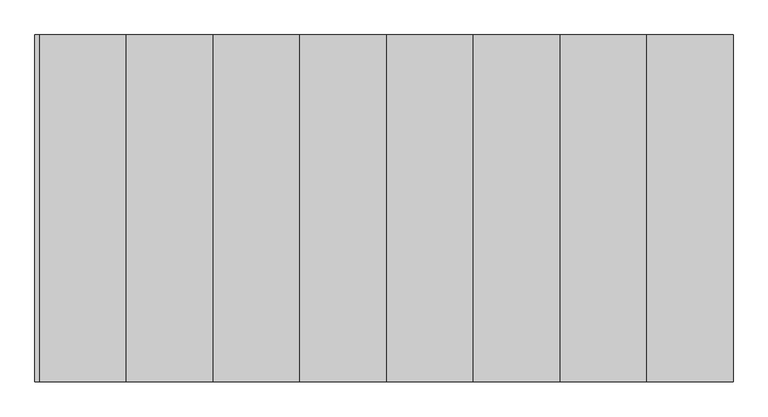
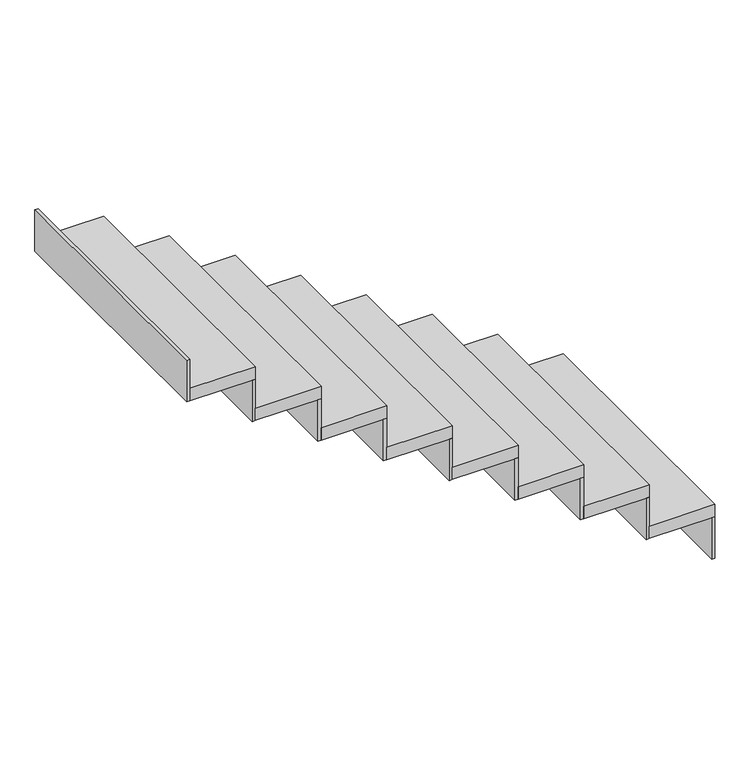
"""IFC4 building model written with IfcOpenShell, lengths in millimetres: stair flight geometry."""

import ifcopenshell
import ifcopenshell.guid

model = None  # the IFC model being written
_history = None  # IfcOwnerHistory: only IFC2X3 demands one
_inside = {}  # id of a spatial element -> (the spatial element, [elements in it])
_under = {}  # id of a project, library or spatial element -> (it, [spatial elements below it])
_declared = {}  # id of a project -> (the project, [libraries it declares])
_typed = {}  # id of a type object -> (the type object, [elements of that type])
_made_of = {}  # id of a material, layer set ... -> (it, [elements and type objects made of it])


def new_model(schema):
    """Start an empty IFC model of exactly this schema.

    Asked for "IFC4X3", IfcOpenShell would pick the latest addendum, in which some entities
    have other attributes; the version numbers below select the first issue.
    IFC2X3 requires an IfcOwnerHistory on every rooted entity: one is made here for all.
    """
    global model, _history
    if schema == "IFC4X3":
        model = ifcopenshell.file(schema_version=(4, 3, 0, 0))
    else:
        model = ifcopenshell.file(schema=schema)
    _inside.clear()
    _under.clear()
    _declared.clear()
    _typed.clear()
    _made_of.clear()
    _history = None
    if model.schema == "IFC2X3":
        org = make("IfcOrganization", Name="unknown")
        user = make(
            "IfcPersonAndOrganization",
            ThePerson=make("IfcPerson", FamilyName="unknown"),
            TheOrganization=org,
        )
        app = make(
            "IfcApplication",
            ApplicationDeveloper=org,
            Version="unknown",
            ApplicationFullName="unknown",
            ApplicationIdentifier="unknown",
        )
        _history = make(
            "IfcOwnerHistory",
            OwningUser=user,
            OwningApplication=app,
            ChangeAction="ADDED",
            CreationDate=0,
        )
    return model


def make(cls, **values):
    """One entity of the class cls with the attributes given. An attribute that is None is left unset."""
    return model.create_entity(
        cls, **{name: value for name, value in values.items() if value is not None}
    )


def rooted(cls, **values):
    """An entity with a GlobalId (a new one), such as an element, a storey or a relation."""
    return make(cls, GlobalId=ifcopenshell.guid.new(), OwnerHistory=_history, **values)


def si_unit(unit_type, name, prefix=None):
    """IfcSIUnit, for example si_unit("LENGTHUNIT", "METRE", prefix="MILLI")."""
    return make("IfcSIUnit", UnitType=unit_type, Prefix=prefix, Name=name)


def assignment(units):
    """IfcUnitAssignment: the units of a project."""
    return None if units is None else make("IfcUnitAssignment", Units=units)


def point(xyz):
    """IfcCartesianPoint."""
    return None if xyz is None else make("IfcCartesianPoint", Coordinates=xyz)


def direction(xyz):
    """IfcDirection."""
    return None if xyz is None else make("IfcDirection", DirectionRatios=xyz)


def frame(location, z_axis=None, x_axis=None):
    """IfcAxis2Placement3D, a coordinate frame: its origin and axes. An axis left out is left unset."""
    return make(
        "IfcAxis2Placement3D",
        Location=point(location),
        Axis=direction(z_axis),
        RefDirection=direction(x_axis),
    )


def origin():
    """The frame at (0, 0, 0) with its axes left unset."""
    return frame((0.0, 0.0, 0.0))


def place(relative_to, where):
    """IfcLocalPlacement: puts the frame where relative to a parent placement (None: the world)."""
    return make(
        "IfcLocalPlacement", PlacementRelTo=relative_to, RelativePlacement=where
    )


def context(
    kind, dimensions, precision=None, world=None, true_north=None, identifier=None
):
    """IfcGeometricRepresentationContext, for example the 3D "Model" context."""
    return make(
        "IfcGeometricRepresentationContext",
        ContextIdentifier=identifier,
        ContextType=kind,
        CoordinateSpaceDimension=dimensions,
        Precision=precision,
        WorldCoordinateSystem=world,
        TrueNorth=true_north,
    )


def project(units=None, contexts=None):
    """IfcProject with its units and contexts."""
    return rooted(
        "IfcProject",
        Name="project",
        RepresentationContexts=contexts,
        UnitsInContext=assignment(units),
    )


def spatial(cls, under=None, at=None, **own):
    """A site, building, storey or space (cls), placed at a placement, below another one or the project."""
    s = rooted(cls, ObjectPlacement=at, **own)
    if under is not None:
        _under.setdefault(under.id(), (under, []))[1].append(s)
    return s


def polyline(points):
    """IfcPolyline through the points."""
    return make("IfcPolyline", Points=[point(p) for p in points])


def outline(outer, holes=None, kind="AREA"):
    """IfcArbitraryClosedProfileDef: a profile drawn as a closed curve; with holes, ...WithVoids."""
    if holes is None:
        return make("IfcArbitraryClosedProfileDef", ProfileType=kind, OuterCurve=outer)
    return make(
        "IfcArbitraryProfileDefWithVoids",
        ProfileType=kind,
        OuterCurve=outer,
        InnerCurves=holes,
    )


def extrude(swept, where, along, depth):
    """IfcExtrudedAreaSolid: the profile swept, set in the frame where, extruded along a direction by depth."""
    return make(
        "IfcExtrudedAreaSolid",
        SweptArea=swept,
        Position=where,
        ExtrudedDirection=direction(along),
        Depth=depth,
    )


def shape(context_of_items, identifier, shape_type, items):
    """IfcShapeRepresentation: the items that make up one representation, for example the "Body"."""
    return make(
        "IfcShapeRepresentation",
        ContextOfItems=context_of_items,
        RepresentationIdentifier=identifier,
        RepresentationType=shape_type,
        Items=items,
    )


def source(mapping_origin, context_of_items, identifier, shape_type, items):
    """IfcRepresentationMap: a shape defined once, which mapped items show again and again."""
    return make(
        "IfcRepresentationMap",
        MappingOrigin=mapping_origin,
        MappedRepresentation=shape(context_of_items, identifier, shape_type, items),
    )


def transform(
    local_origin,
    x_axis=None,
    y_axis=None,
    z_axis=None,
    scale=None,
    scale2=None,
    scale3=None,
    uniform=True,
):
    """IfcCartesianTransformationOperator3D, or its non-uniform kind. x_axis, y_axis, z_axis: its Axis1, 2, 3."""
    if uniform:
        return make(
            "IfcCartesianTransformationOperator3D",
            Axis1=direction(x_axis),
            Axis2=direction(y_axis),
            LocalOrigin=point(local_origin),
            Scale=scale,
            Axis3=direction(z_axis),
        )
    return make(
        "IfcCartesianTransformationOperator3DnonUniform",
        Axis1=direction(x_axis),
        Axis2=direction(y_axis),
        LocalOrigin=point(local_origin),
        Scale=scale,
        Axis3=direction(z_axis),
        Scale2=scale2,
        Scale3=scale3,
    )


def mapped(mapping_source, mapping_target):
    """IfcMappedItem: shows the shape of a source again, moved by a transform."""
    return make(
        "IfcMappedItem", MappingSource=mapping_source, MappingTarget=mapping_target
    )


def made_of(thing, what):
    """Note that an element or type object is made of a material, layer set ...; save() writes the relation."""
    if what is not None:
        _made_of.setdefault(what.id(), (what, []))[1].append(thing)
    return thing


def element(
    cls,
    number,
    at=None,
    inside=None,
    cuts=None,
    type_object=None,
    material=None,
    context=None,
    identifier="Body",
    shape_type=None,
    held_by="IfcProductDefinitionShape",
    body=None,
    shapes=None,
    **own,
):
    """One element of the class cls, such as IfcWall. Its Tag is "e" and its number.

    at: its placement. inside: the storey or other place that contains it. cuts: it is an
    opening in that element (IfcRelVoidsElement). A single representation is given by context,
    identifier, shape_type and body (its items); several are given by shapes. held_by: the class
    of the entity that holds the representations. save() writes the other relations.
    """
    e = rooted(cls, Tag="e%d" % number, ObjectPlacement=at, **own)
    if body is not None:
        shapes = [shape(context, identifier, shape_type, body)]
    if shapes is not None:
        e.Representation = make(held_by, Representations=shapes)
    if inside is not None:
        _inside.setdefault(inside.id(), (inside, []))[1].append(e)
    if cuts is not None:
        rooted(
            "IfcRelVoidsElement", RelatingBuildingElement=cuts, RelatedOpeningElement=e
        )
    if type_object is not None:
        _typed.setdefault(type_object.id(), (type_object, []))[1].append(e)
    return made_of(e, material)


def aggregate(whole, parts):
    """IfcRelAggregates: a whole, such as a stair, and the parts it consists of."""
    return rooted("IfcRelAggregates", RelatingObject=whole, RelatedObjects=parts)


def save(model, path):
    """Write the relations noted so far, then the file.

    IfcRelAggregates (storeys below a building ...), IfcRelContainedInSpatialStructure (elements
    in a storey), IfcRelDefinesByType, IfcRelAssociatesMaterial and IfcRelDeclares: one each for
    every whole, place, type object, material and project.
    """
    for whole, parts in _under.values():
        aggregate(whole, parts)
    for where, things in _inside.values():
        rooted(
            "IfcRelContainedInSpatialStructure",
            RelatedElements=things,
            RelatingStructure=where,
        )
    for kind, things in _typed.values():
        rooted("IfcRelDefinesByType", RelatedObjects=things, RelatingType=kind)
    for what, things in _made_of.values():
        rooted("IfcRelAssociatesMaterial", RelatedObjects=things, RelatingMaterial=what)
    for by, libraries in _declared.values():
        rooted("IfcRelDeclares", RelatingContext=by, RelatedDefinitions=libraries)
    model.write(path)


def stair_flight_f3270307(model_context):
    return source(origin(), model_context, "Body", "SweptSolid", [
        extrude(outline(polyline([(5264.0556606, 2510.81281), (5276.5556606, 2510.81281), (5276.5556606, 1510.81281), (5264.0556606, 1510.81281), (5264.0556606, 2510.81281)])), frame((0.0, 0.0, 4750.0), z_axis=(0.0, 0.0, 1.0), x_axis=(1.0, 0.0, 0.0)), (0.0, 0.0, 1.0), 166.6666667),
        extrude(outline(polyline([(5026.5556606, 1510.81281), (5026.5556606, 2510.81281), (5276.5556606, 2510.81281), (5276.5556606, 1510.81281), (5026.5556606, 1510.81281)])), frame((0.0, 0.0, 4916.6666667), z_axis=(0.0, 0.0, 1.0), x_axis=(1.0, 0.0, 0.0)), (0.0, 0.0, 1.0), 50.0),
        extrude(outline(polyline([(5014.0556606, 2510.81281), (5026.5556606, 2510.81281), (5026.5556606, 1510.81281), (5014.0556606, 1510.81281), (5014.0556606, 2510.81281)])), frame((0.0, 0.0, 4916.6666667), z_axis=(0.0, 0.0, 1.0), x_axis=(1.0, 0.0, 0.0)), (0.0, 0.0, 1.0), 166.6666667),
        extrude(outline(polyline([(4776.5556606, 1510.81281), (4776.5556606, 2510.81281), (5026.5556606, 2510.81281), (5026.5556606, 1510.81281), (4776.5556606, 1510.81281)])), frame((0.0, 0.0, 5083.3333333), z_axis=(0.0, 0.0, 1.0), x_axis=(1.0, 0.0, 0.0)), (0.0, 0.0, 1.0), 50.0),
        extrude(outline(polyline([(4764.0556606, 2510.81281), (4776.5556606, 2510.81281), (4776.5556606, 1510.81281), (4764.0556606, 1510.81281), (4764.0556606, 2510.81281)])), frame((0.0, 0.0, 5083.3333333), z_axis=(0.0, 0.0, 1.0), x_axis=(1.0, 0.0, 0.0)), (0.0, 0.0, 1.0), 166.6666667),
        extrude(outline(polyline([(4526.5556606, 1510.81281), (4526.5556606, 2510.81281), (4776.5556606, 2510.81281), (4776.5556606, 1510.81281), (4526.5556606, 1510.81281)])), frame((0.0, 0.0, 5250.0), z_axis=(0.0, 0.0, 1.0), x_axis=(1.0, 0.0, 0.0)), (0.0, 0.0, 1.0), 50.0),
        extrude(outline(polyline([(4514.0556606, 2510.81281), (4526.5556606, 2510.81281), (4526.5556606, 1510.81281), (4514.0556606, 1510.81281), (4514.0556606, 2510.81281)])), frame((0.0, 0.0, 5250.0), z_axis=(0.0, 0.0, 1.0), x_axis=(1.0, 0.0, 0.0)), (0.0, 0.0, 1.0), 166.6666667),
        extrude(outline(polyline([(4276.5556606, 1510.81281), (4276.5556606, 2510.81281), (4526.5556606, 2510.81281), (4526.5556606, 1510.81281), (4276.5556606, 1510.81281)])), frame((0.0, 0.0, 5416.6666667), z_axis=(0.0, 0.0, 1.0), x_axis=(1.0, 0.0, 0.0)), (0.0, 0.0, 1.0), 50.0),
        extrude(outline(polyline([(4264.0556606, 2510.81281), (4276.5556606, 2510.81281), (4276.5556606, 1510.81281), (4264.0556606, 1510.81281), (4264.0556606, 2510.81281)])), frame((0.0, 0.0, 5416.6666667), z_axis=(0.0, 0.0, 1.0), x_axis=(1.0, 0.0, 0.0)), (0.0, 0.0, 1.0), 166.6666667),
        extrude(outline(polyline([(4026.5556606, 1510.81281), (4026.5556606, 2510.81281), (4276.5556606, 2510.81281), (4276.5556606, 1510.81281), (4026.5556606, 1510.81281)])), frame((0.0, 0.0, 5583.3333333), z_axis=(0.0, 0.0, 1.0), x_axis=(1.0, 0.0, 0.0)), (0.0, 0.0, 1.0), 50.0),
        extrude(outline(polyline([(4014.0556606, 2510.81281), (4026.5556606, 2510.81281), (4026.5556606, 1510.81281), (4014.0556606, 1510.81281), (4014.0556606, 2510.81281)])), frame((0.0, 0.0, 5583.3333333), z_axis=(0.0, 0.0, 1.0), x_axis=(1.0, 0.0, 0.0)), (0.0, 0.0, 1.0), 166.6666667),
        extrude(outline(polyline([(3776.5556606, 1510.81281), (3776.5556606, 2510.81281), (4026.5556606, 2510.81281), (4026.5556606, 1510.81281), (3776.5556606, 1510.81281)])), frame((0.0, 0.0, 5750.0), z_axis=(0.0, 0.0, 1.0), x_axis=(1.0, 0.0, 0.0)), (0.0, 0.0, 1.0), 50.0),
        extrude(outline(polyline([(3764.0556606, 2510.81281), (3776.5556606, 2510.81281), (3776.5556606, 1510.81281), (3764.0556606, 1510.81281), (3764.0556606, 2510.81281)])), frame((0.0, 0.0, 5750.0), z_axis=(0.0, 0.0, 1.0), x_axis=(1.0, 0.0, 0.0)), (0.0, 0.0, 1.0), 166.6666667),
        extrude(outline(polyline([(3526.5556606, 1510.81281), (3526.5556606, 2510.81281), (3776.5556606, 2510.81281), (3776.5556606, 1510.81281), (3526.5556606, 1510.81281)])), frame((0.0, 0.0, 5916.6666667), z_axis=(0.0, 0.0, 1.0), x_axis=(1.0, 0.0, 0.0)), (0.0, 0.0, 1.0), 50.0),
        extrude(outline(polyline([(3514.0556606, 2510.81281), (3526.5556606, 2510.81281), (3526.5556606, 1510.81281), (3514.0556606, 1510.81281), (3514.0556606, 2510.81281)])), frame((0.0, 0.0, 5916.6666667), z_axis=(0.0, 0.0, 1.0), x_axis=(1.0, 0.0, 0.0)), (0.0, 0.0, 1.0), 166.6666667),
        extrude(outline(polyline([(3264.0556606, 2510.81281), (3276.5556606, 2510.81281), (3276.5556606, 1510.81281), (3264.0556606, 1510.81281), (3264.0556606, 2510.81281)])), frame((0.0, 0.0, 6083.3333333), z_axis=(0.0, 0.0, 1.0), x_axis=(1.0, 0.0, 0.0)), (0.0, 0.0, 1.0), 166.6666667),
        extrude(outline(polyline([(3276.5556606, 1510.81281), (3276.5556606, 2510.81281), (3526.5556606, 2510.81281), (3526.5556606, 1510.81281), (3276.5556606, 1510.81281)])), frame((0.0, 0.0, 6083.3333333), z_axis=(0.0, 0.0, 1.0), x_axis=(1.0, 0.0, 0.0)), (0.0, 0.0, 1.0), 50.0),
    ])


if __name__ == "__main__":
    model = new_model("IFC4")
    model_context = context("Model", 3, world=origin())
    ifc_project = project(units=[si_unit("LENGTHUNIT", "METRE", prefix="MILLI")], contexts=[model_context])
    site = spatial("IfcSite", under=ifc_project)
    building = spatial("IfcBuilding", under=site)
    placement = place(None, origin())
    stair_flight_shape = stair_flight_f3270307(model_context)
    element("IfcStairFlight", 1, at=placement, inside=building, context=model_context, shape_type="MappedRepresentation", body=[
        mapped(stair_flight_shape, transform((0.0, 0.0, 0.0), x_axis=(1.0, 0.0, 0.0), y_axis=(0.0, 1.0, 0.0), z_axis=(0.0, 0.0, 1.0))),
    ])
    save(model, "model.ifc")
